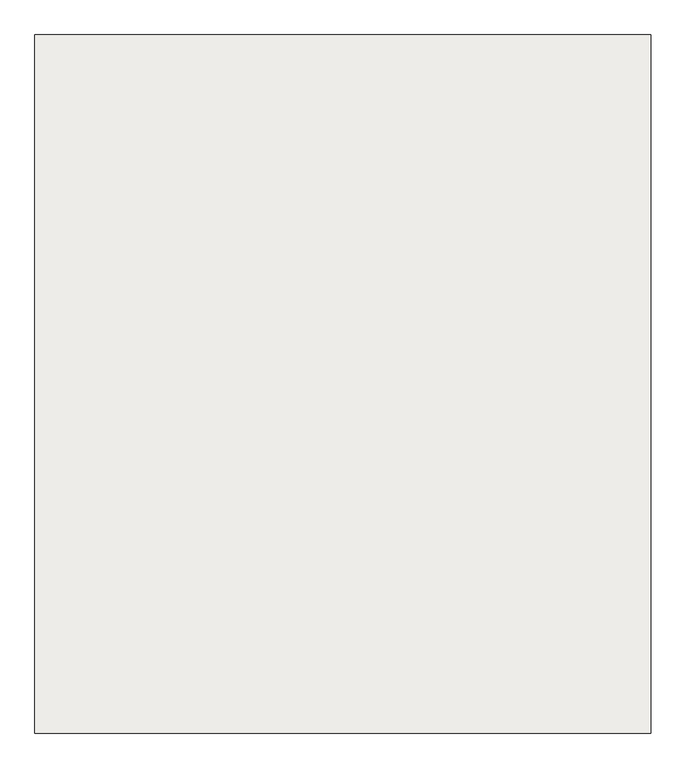
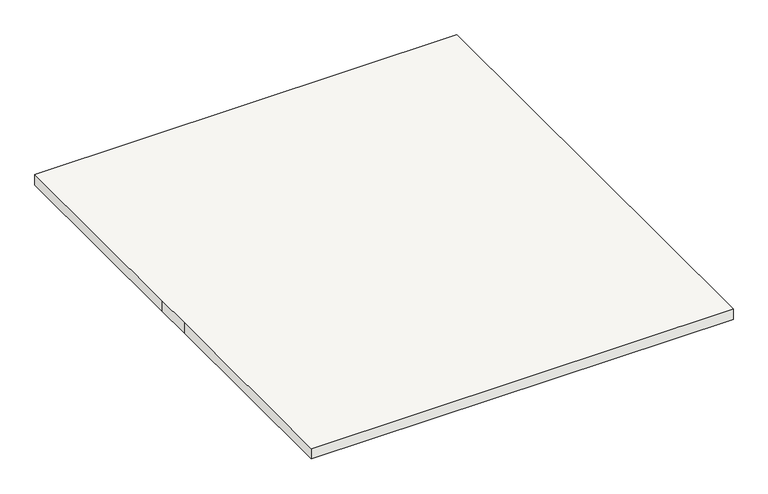
"""IFC4 building model written with IfcOpenShell, lengths in millimetres: slab geometry."""

from ifc_helpers import new_model, si_unit, frame, origin, place, context, project, spatial, polyline, outline, extrude, source, transform, mapped, element, save


def slab_0549d9b8(model_context):
    return source(origin(), model_context, "Body", "SweptSolid", [
        extrude(outline(polyline([(5276.5556606, 3685.7983707), (7194.8909543, 3685.7983707), (7194.8909543, 1510.81281), (5276.5556606, 1510.81281), (5276.5556606, 2510.81281), (5276.5556606, 2685.7983707), (5276.5556606, 3685.7983707)])), frame((0.0, 0.0, 4750.0), z_axis=(0.0, 0.0, 1.0), x_axis=(1.0, 0.0, 0.0)), (0.0, 0.0, 1.0), 50.0),
    ])


if __name__ == "__main__":
    model = new_model("IFC4")
    model_context = context("Model", 3, world=origin())
    ifc_project = project(units=[si_unit("LENGTHUNIT", "METRE", prefix="MILLI")], contexts=[model_context])
    site = spatial("IfcSite", under=ifc_project)
    building = spatial("IfcBuilding", under=site)
    placement = place(None, origin())
    slab_shape = slab_0549d9b8(model_context)
    element("IfcSlab", 1, at=placement, inside=building, context=model_context, shape_type="MappedRepresentation", body=[
        mapped(slab_shape, transform((0.0, 0.0, 0.0), x_axis=(1.0, 0.0, 0.0), y_axis=(0.0, 1.0, 0.0), z_axis=(0.0, 0.0, 1.0))),
    ])
    save(model, "model.ifc")

# Revit data of these elements
# Project information
#   项目发布日期 = "出图日期"
#   项目状态 = "项目状态"
#   客户姓名 = "所有者"
#   项目地址 = "请在此处输入地址"
#   项目名称 = "项目名称"
#   项目编号 = "项目编号"
